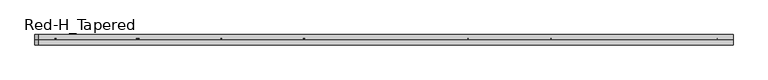
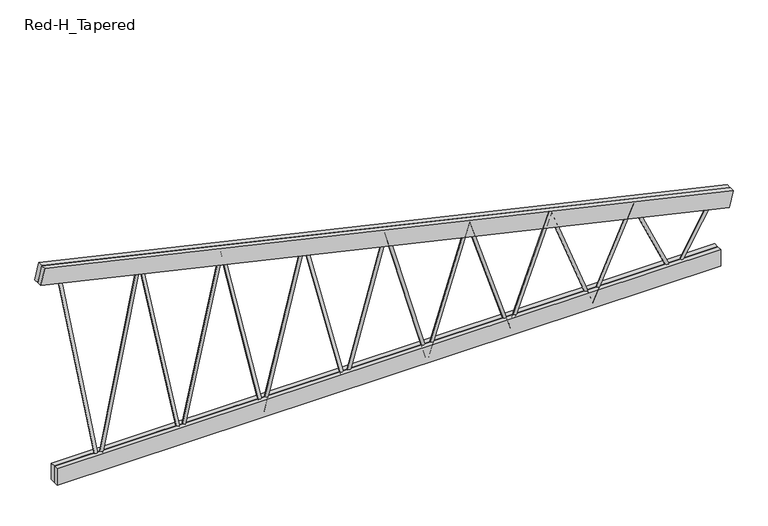
"""IFC4 building model written with IfcOpenShell, lengths in millimetres: beam geometry, Construction_Frames_RedBuilt_Openweb_Red-H_Tapered : Red-H_Tapered."""

from ifc_helpers import new_model, si_unit, point, frame, origin, origin_2d, place, context, project, spatial, polyline, circle_curve, trimmed, segment, composite_curve, outline, extrude, source, transform, mapped, element, save


def red_h_tapered_bf32dc33(model_context):
    return source(origin(), model_context, "Body", "SweptSolid", [
        extrude(outline(composite_curve([segment(trimmed(circle_curve(origin_2d(), 12.7), [point((0.0, 12.6999999))], [point((0.0, -12.7000001))], False, "CARTESIAN"), True, "CONTINUOUS"), segment(trimmed(circle_curve(origin_2d(), 12.7), [point((0.0, -12.7000001))], [point((0.0, 12.6999999))], False, "CARTESIAN"), True, "CONTINUOUS")], self_intersect=False)), frame((-332.2835937, 0.0, -367.0101562), z_axis=(-0.24049924199375627, 0.0, 0.9706493262761937), x_axis=(0.0, -1.0, 0.0)), (0.0, 0.0, 1.0), 1381.6409191),
        extrude(outline(composite_curve([segment(trimmed(circle_curve(origin_2d(), 12.7), [point((0.0, -12.7))], [point((0.0, 12.7))], False, "CARTESIAN"), True, "CONTINUOUS"), segment(trimmed(circle_curve(origin_2d(), 12.7), [point((0.0, 12.7))], [point((0.0, -12.7))], False, "CARTESIAN"), True, "CONTINUOUS")], self_intersect=False)), frame((-996.8507812, 0.0, -367.0101562), z_axis=(0.24049924199375522, 0.0, 0.9706493262761939), x_axis=(0.0, -1.0, 0.0)), (0.0, 0.0, 1.0), 1381.6409191),
        extrude(outline(composite_curve([segment(trimmed(circle_curve(origin_2d(), 12.7), [point((0.0, 12.6999999))], [point((0.0, -12.7))], False, "CARTESIAN"), True, "CONTINUOUS"), segment(trimmed(circle_curve(origin_2d(), 12.7), [point((0.0, -12.7))], [point((0.0, 12.6999999))], False, "CARTESIAN"), True, "CONTINUOUS")], self_intersect=False)), frame((-996.8507812, 0.0, -367.0101562), z_axis=(-0.21731956167576924, 0.0, 0.9761005112758888), x_axis=(0.0, -1.0, 0.0)), (0.0, 0.0, 1.0), 1529.0091292),
        extrude(outline(composite_curve([segment(trimmed(circle_curve(origin_2d(), 12.7), [point((0.0, -12.7))], [point((0.0, 12.6999999))], False, "CARTESIAN"), True, "CONTINUOUS"), segment(trimmed(circle_curve(origin_2d(), 12.7), [point((0.0, 12.6999999))], [point((0.0, -12.7))], False, "CARTESIAN"), True, "CONTINUOUS")], self_intersect=False)), frame((-1661.4179687, 0.0, -367.0101562), z_axis=(0.21731956167577737, 0.0, 0.976100511275887), x_axis=(0.0, -1.0, 0.0)), (0.0, 0.0, 1.0), 1529.0091292),
        extrude(outline(composite_curve([segment(trimmed(circle_curve(origin_2d(), 12.7), [point((0.0, 12.6999999))], [point((0.0, -12.7))], False, "CARTESIAN"), True, "CONTINUOUS"), segment(trimmed(circle_curve(origin_2d(), 12.7), [point((0.0, -12.7))], [point((0.0, 12.6999999))], False, "CARTESIAN"), True, "CONTINUOUS")], self_intersect=False)), frame((-1661.4179687, 0.0, -367.0101562), z_axis=(-0.19813084067481326, 0.0, 0.9801755811962936), x_axis=(0.0, -1.0, 0.0)), (0.0, 0.0, 1.0), 1677.091727),
        extrude(outline(composite_curve([segment(trimmed(circle_curve(origin_2d(), 12.7), [point((0.0, -12.7))], [point((0.0, 12.6999999))], False, "CARTESIAN"), True, "CONTINUOUS"), segment(trimmed(circle_curve(origin_2d(), 12.7), [point((0.0, 12.6999999))], [point((0.0, -12.7))], False, "CARTESIAN"), True, "CONTINUOUS")], self_intersect=False)), frame((-2325.9851562, 0.0, -367.0101562), z_axis=(0.1981308406748069, 0.0, 0.9801755811962949), x_axis=(0.0, -1.0, 0.0)), (0.0, 0.0, 1.0), 1677.091727),
        extrude(outline(composite_curve([segment(trimmed(circle_curve(origin_2d(), 12.7), [point((0.0, 12.6999999))], [point((0.0, -12.7000001))], False, "CARTESIAN"), True, "CONTINUOUS"), segment(trimmed(circle_curve(origin_2d(), 12.7), [point((0.0, -12.7000001))], [point((0.0, 12.6999999))], False, "CARTESIAN"), True, "CONTINUOUS")], self_intersect=False)), frame((-2325.9851562, 0.0, -367.0101562), z_axis=(-0.1820019081589403, 0.0, 0.9832981772720342), x_axis=(0.0, -1.0, 0.0)), (0.0, 0.0, 1.0), 1825.7148901),
        extrude(outline(composite_curve([segment(trimmed(circle_curve(origin_2d(), 12.7), [point((0.0, 12.7000001))], [point((0.0, -12.7))], False, "CARTESIAN"), True, "CONTINUOUS"), segment(trimmed(circle_curve(origin_2d(), 12.7), [point((0.0, -12.7))], [point((0.0, 12.7000001))], False, "CARTESIAN"), True, "CONTINUOUS")], self_intersect=False)), frame((2325.9851562, 0.0, -367.0101562), z_axis=(0.4944050285555307, 0.0, 0.8692316536683445), x_axis=(0.0, -1.0, 0.0)), (0.0, 0.0, 1.0), 672.0878117),
        extrude(outline(composite_curve([segment(trimmed(circle_curve(origin_2d(), 12.7), [point((0.0, -12.6999999))], [point((0.0, 12.7))], False, "CARTESIAN"), True, "CONTINUOUS"), segment(trimmed(circle_curve(origin_2d(), 12.7), [point((0.0, 12.7))], [point((0.0, -12.6999999))], False, "CARTESIAN"), True, "CONTINUOUS")], self_intersect=False)), frame((2325.9851562, 0.0, -367.0101562), z_axis=(-0.41167643679554905, 0.0, 0.9113300781754766), x_axis=(0.0, -1.0, 0.0)), (0.0, 0.0, 1.0), 807.1474684),
        extrude(outline(composite_curve([segment(trimmed(circle_curve(origin_2d(), 12.7), [point((0.0, 12.7))], [point((0.0, -12.6999999))], False, "CARTESIAN"), True, "CONTINUOUS"), segment(trimmed(circle_curve(origin_2d(), 12.7), [point((0.0, -12.6999999))], [point((0.0, 12.7))], False, "CARTESIAN"), True, "CONTINUOUS")], self_intersect=False)), frame((1661.4179687, 0.0, -367.0101562), z_axis=(0.41167643679554944, 0.0, 0.9113300781754765), x_axis=(0.0, -1.0, 0.0)), (0.0, 0.0, 1.0), 807.1474684),
        extrude(outline(composite_curve([segment(trimmed(circle_curve(origin_2d(), 12.7), [point((0.0, -12.7))], [point((0.0, 12.7))], False, "CARTESIAN"), True, "CONTINUOUS"), segment(trimmed(circle_curve(origin_2d(), 12.7), [point((0.0, 12.7))], [point((0.0, -12.7))], False, "CARTESIAN"), True, "CONTINUOUS")], self_intersect=False)), frame((1661.4179687, 0.0, -367.0101562), z_axis=(-0.35082284427885274, 0.0, 0.9364418465297757), x_axis=(0.0, -1.0, 0.0)), (0.0, 0.0, 1.0), 947.1549506),
        extrude(outline(composite_curve([segment(trimmed(circle_curve(origin_2d(), 12.7), [point((0.0, 12.7000001))], [point((0.0, -12.6999999))], False, "CARTESIAN"), True, "CONTINUOUS"), segment(trimmed(circle_curve(origin_2d(), 12.7), [point((0.0, -12.6999999))], [point((0.0, 12.7000001))], False, "CARTESIAN"), True, "CONTINUOUS")], self_intersect=False)), frame((996.8507812, 0.0, -367.0101562), z_axis=(0.35082284427885174, 0.0, 0.936441846529776), x_axis=(0.0, -1.0, 0.0)), (0.0, 0.0, 1.0), 947.1549506),
        extrude(outline(composite_curve([segment(trimmed(circle_curve(origin_2d(), 12.7), [point((0.0, -12.6999999))], [point((0.0, 12.7))], False, "CARTESIAN"), True, "CONTINUOUS"), segment(trimmed(circle_curve(origin_2d(), 12.7), [point((0.0, 12.7))], [point((0.0, -12.6999999))], False, "CARTESIAN"), True, "CONTINUOUS")], self_intersect=False)), frame((996.8507812, 0.0, -367.0101562), z_axis=(-0.3047898211881548, 0.0, 0.9524196369773634), x_axis=(0.0, -1.0, 0.0)), (0.0, 0.0, 1.0), 1090.2056783),
        extrude(outline(composite_curve([segment(trimmed(circle_curve(origin_2d(), 12.7), [point((0.0, 12.6999999))], [point((0.0, -12.7))], False, "CARTESIAN"), True, "CONTINUOUS"), segment(trimmed(circle_curve(origin_2d(), 12.7), [point((0.0, -12.7))], [point((0.0, 12.6999999))], False, "CARTESIAN"), True, "CONTINUOUS")], self_intersect=False)), frame((332.2835938, 0.0, -367.0101562), z_axis=(0.30478982118815523, 0.0, 0.9524196369773633), x_axis=(0.0, -1.0, 0.0)), (0.0, 0.0, 1.0), 1090.2056783),
        extrude(outline(composite_curve([segment(trimmed(circle_curve(origin_2d(), 12.7), [point((0.0, -12.7000001))], [point((0.0, 12.7))], False, "CARTESIAN"), True, "CONTINUOUS"), segment(trimmed(circle_curve(origin_2d(), 12.7), [point((0.0, 12.7))], [point((0.0, -12.7000001))], False, "CARTESIAN"), True, "CONTINUOUS")], self_intersect=False)), frame((332.2835938, 0.0, -367.0101562), z_axis=(-0.2690026538242675, 0.0, 0.9631394355105087), x_axis=(0.0, -1.0, 0.0)), (0.0, 0.0, 1.0), 1235.242809),
        extrude(outline(composite_curve([segment(trimmed(circle_curve(origin_2d(), 12.7), [point((0.0, -12.7000001))], [point((0.0, 12.7))], False, "CARTESIAN"), True, "CONTINUOUS"), segment(trimmed(circle_curve(origin_2d(), 12.7), [point((0.0, 12.7))], [point((0.0, -12.7000001))], False, "CARTESIAN"), True, "CONTINUOUS")], self_intersect=False)), frame((-332.2835937, 0.0, -367.0101562), z_axis=(0.26900265382424515, 0.0, 0.963139435510515), x_axis=(0.0, -1.0, 0.0)), (0.0, 0.0, 1.0), 1235.242809),
        extrude(outline(polyline([(-2683.66875, -41.275), (-2683.66875, -3.175), (2683.66875, -3.175), (2683.66875, -41.275), (-2683.66875, -41.275)])), frame((0.0, 0.0, -386.0601562), z_axis=(0.0, 0.0, 1.0), x_axis=(1.0, 0.0, 0.0)), (0.0, 0.0, 1.0), 139.7),
        extrude(outline(polyline([(-2683.66875, 3.175), (-2683.66875, 41.275), (2683.66875, 41.275), (2683.66875, 3.175), (-2683.66875, 3.175)])), frame((0.0, 0.0, -386.0601562), z_axis=(0.0, 0.0, 1.0), x_axis=(1.0, 0.0, 0.0)), (0.0, 0.0, 1.0), 139.7),
        extrude(outline(polyline([(0.0, -38.1), (0.0, 0.0), (5716.3106396, 0.0), (5716.3106396, -38.1), (0.0, -38.1)])), frame((-2816.6164498, -3.175, 1370.1023702), z_axis=(0.22439298366750388, 0.0, 0.9744987372392), x_axis=(0.9744987372392, 0.0, -0.22439298366750388)), (0.0, 0.0, 1.0), 139.7),
        extrude(outline(polyline([(0.0, -38.1), (0.0, 0.0), (5716.3106396, 0.0), (5716.3106396, -38.1), (0.0, -38.1)])), frame((-2816.6164498, 41.275, 1370.1023702), z_axis=(0.22439298366750388, 0.0, 0.9744987372392), x_axis=(0.9744987372392, 0.0, -0.22439298366750388)), (0.0, 0.0, 1.0), 139.7),
    ])


if __name__ == "__main__":
    model = new_model("IFC4")
    model_context = context("Model", 3, world=origin())
    ifc_project = project(units=[si_unit("LENGTHUNIT", "METRE", prefix="MILLI")], contexts=[model_context])
    site = spatial("IfcSite", under=ifc_project)
    building = spatial("IfcBuilding", under=site)
    placement = place(None, origin())
    red_h_tapered_shape = red_h_tapered_bf32dc33(model_context)
    element("IfcBeam", 1, ObjectType="Construction_Frames_RedBuilt_Openweb_Red-H_Tapered : Red-H_Tapered", at=placement, inside=building, context=model_context, shape_type="MappedRepresentation", body=[
        mapped(red_h_tapered_shape, transform((0.0, 0.0, 0.0), x_axis=(1.0, 0.0, 0.0), y_axis=(0.0, 1.0, 0.0), z_axis=(0.0, 0.0, 1.0))),
    ])
    save(model, "model.ifc")

# Revit data of these elements
# Type "Construction_Frames_RedBuilt_Openweb_Red-H_Tapered : Red-H_Tapered"
#   Youtube clip = ""
#   Weight Net (Kg) = "0"
#   Webs = "Up to 2\" diameter tubular steel"
#   Uniformat II Description = ""
#   Uniformat II Code = ""
#   Uniclass 2015 Name = "Softwood trusses"
#   Uniclass 2015 Code = "Pr_20_85_90_81"
#   Uniclass 2.0 Description = "Structural Framing Systems"
#   Uniclass 2.0 Code = "SS-15-10-75"
#   Uniclass 1.4 Description = "Trusses"
#   Uniclass 1.4 Code = "L3523"
#   UNSPSC Code = "30103606"
#   Technical description = "http://www.redbuilt.com/reference/literature-and-other-resources"
#   Region South America = "None"
#   Region Oceania = "None"
#   Region North America = "US"
#   Region Middle East = "None"
#   Region Europe = "None"
#   Region Asia = "None"
#   Region Antarctica = "None"
#   Region Africa = "None"
#   QR code = "http://bimobject.com/redbuilt/product/redbuilt-0003"
#   Product url = "http://www.redbuilt.com/products/default.aspx?id=2"
#   Product group = "Wood Trusses"
#   Product family = "Construction"
#   Product data url = "https://bimobject.com/redbuilt/product/redbuilt-0003"
#   Product certification = ""
#   Product SKU = "redbuilt-0003"
#   Product Page URL = "http://www.redbuilt.com/commercial-systems/red-m-red-h-open-web-trusses"
#   Product Guid = "2c5793f2-6ffb-4665-b825-cf90c048e711"
#   Product Documentation Link = "http://www.redbuilt.com/documents/OW_Guide_2017_07_LowRes_wLinks.pdf"
#   OmniClass Description = "Wood Trusses"
#   OmniClass Code = "23-13 35 19 13 17"
#   NBS Reference Description = ""
#   NBS Reference Code = ""
#   Material secondary = "Steel"
#   Material main = "Wood"
#   Masterformat 2014 Description = "Metal-Web Wood Joists"
#   Masterformat 2014 Code = "06 17 36"
#   Manufacturer name = "RedBuilt"
#   Manufacturer country = "United States"
#   Installation instructions = "http://www.redbuilt.com/documents/Installation_Sheets_Open-Web.pdf"
#   IFC Classification = ""
#   EAN code = ""
#   Design country = "United States"
#   Product Information = "http://redbuilt.com/products/default.aspx?id=2"
#   Model = "Red-H-Tapered"
#   Manufacturer URL = "http://redbuilt.com/"
#   Manufacturer = "RedBuilt™"
#   Description = "Open Web Truss"
#   Date of publishing = "8/17/2010"
#   Contact us = "http://redbuilt.com/contact/"
#   Chords = "Double 1½\" x 5½\" MSR lumber"
#   COBIe Type Category = ""
#   Brand url = "http://www.redbuilt.com"
#   BIMobject main category code = "construction"
#   BIMobject main category = "Construction"
#   BIMobject category code = "construction-frames-trusses"
#   BIMobject category = "Frames & Trusses"
#   Web Radius = 0' - 0 1/2"
#   Web Layout Offset Start [instance default] = 0' - 5"
#   Web Layout Offset End [instance default] = 0' - 5"
#   Web Diameter = 0' - 1"
#   TotalLength [instance default] = 20' - 0"
#   Span Minimum = 4' - 0"
#   Span Maximum = 70' - 0"
#   Span Limit [instance default] = 20' - 0"
#   Nominal width = 0' - 0"
#   Nominal height = 0' - 0"
#   Inner Depth Top [instance default] = 0' - 2.76372"
#   Depth Start [instance default] = 6' - 0"
#   Top Chord Length [instance default] = 20' - 1.19701"
#   TC Extension Start Aux [instance default] = 0' - 0"
#   TC Extension End Aux [instance default] = 0' - 0"
#   T-B Chord Length Difference L [instance default] = 0' - 4"
#   T-B Chord Length Difference [instance default] = 0' - 4"
#   Height 2 [instance default] = 6' - 0"
#   Depth Minimum at Wall = 2' - 0"
#   Depth Maximum at Wall = 6' - 0"
#   Depth Lower End [instance default] = 2' - 0"
#   Depth Higher End [instance default] = 6' - 0"
#   Depth End [instance default] = 2' - 0"
#   Depth 2 [instance default] = 2' - 0"
#   Chord Width = 0' - 3 1/4"
#   Chord Thickness = 0' - 1 1/2"
#   Chord Depth = 0' - 5 1/2"
#   Offset Start [instance default] = 0' - 0"
#   TC Extension Start [instance default] = 0' - 0"
#   End Panel = 0' - 5"
#   Offset End [instance default] = 0' - 0"
#   TC Extension End [instance default] = 0' - 0"
#   Length [instance default] = 20' - 0"
#   Angle [instance default] = 5.71059°
#   Span Limit Warning [instance default] = no
#   Edition number = 1
#   Top Bearing Start [instance default] = yes
#   Top Bearing End [instance default] = yes
#   Bottom Bearing Start [instance default] = no
#   Bottom Bearing End [instance default] = no
#   8 Panels [instance default] = yes
#   16 Panels [instance default] = no
#   12 Panels [instance default] = no
#   Web Material = RedBuilt-Steel, Galvanized
#   Clip Material = RedBuilt-Steel, Galvanized
#   Chords Material = RedBuilt-MSR
#   URL = ""
#   Assembly Code = ""
# Element 1 (IfcBeam, "Construction_Frames_RedBuilt_Openweb_Red-H_Tapered : Red-H_Tapered")
#   TotalLength = 18' - 3 5/16"
#   Span Limit = 18' - 3 5/16"
#   Inner Depth Top = 0' - 2.82196"
#   Top Chord Length = 18' - 9.0516"
#   Depth 2 = 4' - 2 1/2"
#   Angle = 12.9672°
#   Materials on its faces: "RedBuilt-Steel, Galvanized", "RedBuilt-MSR"
# Materials
#   "RedBuilt-Steel, Galvanized": class "Metal", colour RGB 164 172 176, transparency 0, Manufacturer = "RedBuilt. LLC", Comments = "Openweb Metal Web", URL = "http://www.redbuilt.com/", Description = "Galvanized steel", Cost = 0
#   "RedBuilt-MSR": class "Wood", colour RGB 213 182 136, transparency 0, Manufacturer = "RedBuilt, LLC", URL = "http://www.redbuilt.com/", Cost = 0
